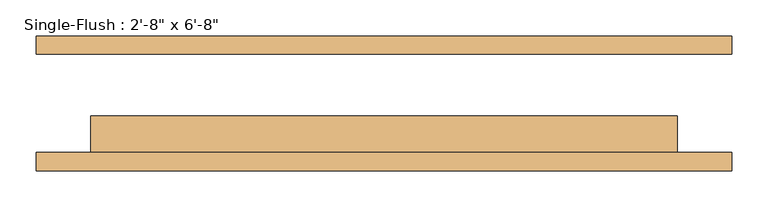
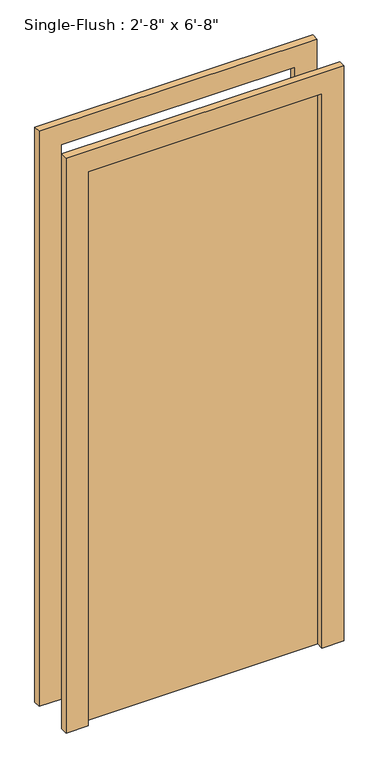
"""IFC4 building model written with IfcOpenShell, lengths in millimetres: door geometry."""

from ifc_helpers import new_model, si_unit, frame, origin, origin_with_axes, place, context, project, spatial, polyline, outline, extrude, source, transform, mapped, element, save


def door_a239bf7e(model_context):
    return source(origin(), model_context, "Body", "SweptSolid", [
        extrude(outline(polyline([(2108.2, -482.6), (0.0, -482.6), (0.0, -406.4), (2032.0, -406.4), (2032.0, 406.4), (0.0, 406.4), (0.0, 482.6), (2108.2, 482.6), (2108.2, -482.6)])), frame((0.0, -93.6625, 0.0), z_axis=(0.0, 1.0, 0.0), x_axis=(0.0, 0.0, 1.0)), (0.0, 0.0, 1.0), 25.4),
        extrude(outline(polyline([(2108.2, 482.6), (2108.2, -482.6), (0.0, -482.6), (0.0, -406.4), (2032.0, -406.4), (2032.0, 406.4), (0.0, 406.4), (0.0, 482.6), (2108.2, 482.6)])), frame((0.0, 68.2625, 0.0), z_axis=(0.0, 1.0, 0.0), x_axis=(0.0, 0.0, 1.0)), (0.0, 0.0, 1.0), 25.4),
        extrude(outline(polyline([(406.4, -17.4625), (406.4, -68.2625), (-406.4, -68.2625), (-406.4, -17.4625), (406.4, -17.4625)])), origin_with_axes(), (0.0, 0.0, 1.0), 2032.0),
    ])


if __name__ == "__main__":
    model = new_model("IFC4")
    model_context = context("Model", 3, world=origin())
    ifc_project = project(units=[si_unit("LENGTHUNIT", "METRE", prefix="MILLI")], contexts=[model_context])
    site = spatial("IfcSite", under=ifc_project)
    building = spatial("IfcBuilding", under=site)
    placement = place(None, origin())
    door_shape = door_a239bf7e(model_context)
    element("IfcDoor", 1, ObjectType="Single-Flush : 2'-8\" x 6'-8\"", at=placement, inside=building, context=model_context, shape_type="MappedRepresentation", body=[
        mapped(door_shape, transform((0.0, 0.0, 0.0), x_axis=(1.0, 0.0, 0.0), y_axis=(0.0, 1.0, 0.0), z_axis=(0.0, 0.0, 1.0))),
    ])
    save(model, "model.ifc")

# Revit data of these elements
# Type "Single-Flush : 2'-8\" x 6'-8\""
#   Type Mark = "11"
#   Construction Type Id = "MDOOR"
#   Assembly Code = "C1020"
#   Analytic Construction = "Metal"
#   Thickness = 0' - 2"
#   Heat Transfer Coefficient (U) = 3.7021 W/(m²·K)
#   Height = 6' - 8"
#   Trim Projection Ext = 0' - 1"
#   Trim Projection Int = 0' - 1"
#   Trim Width = 0' - 3"
#   Width = 2' - 8"
#   Door Material = Door - Panel
#   Frame Material = Door - Frame
#   Visual Light Transmittance = 0
#   Solar Heat Gain Coefficient = 0
#   Function = (empty or 0)
#   Wall Closure = (empty or 0)
# Element 1 (IfcDoor, "Single-Flush : 2'-8\" x 6'-8\"")
#   Materials on its faces: "Door - Frame", "Door - Panel"
# Materials
#   "Door - Panel": class "Wood", colour RGB 210 159 95, transparency 0, Cost = 0
#   "Door - Frame": class "Miscellaneous", colour RGB 118 70 51, transparency 0, Cost = 0
